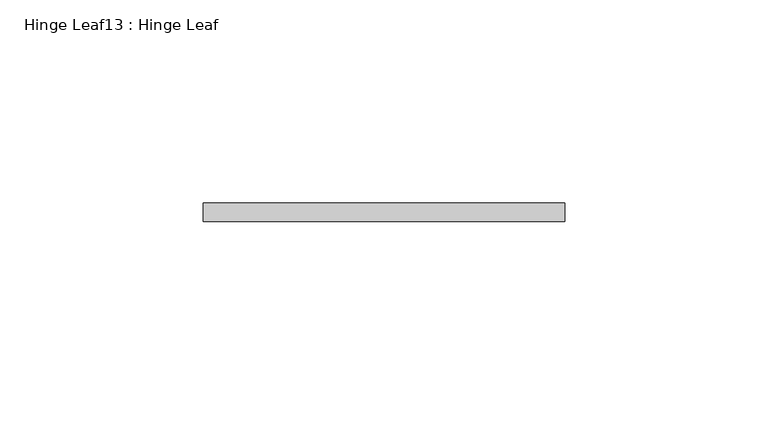
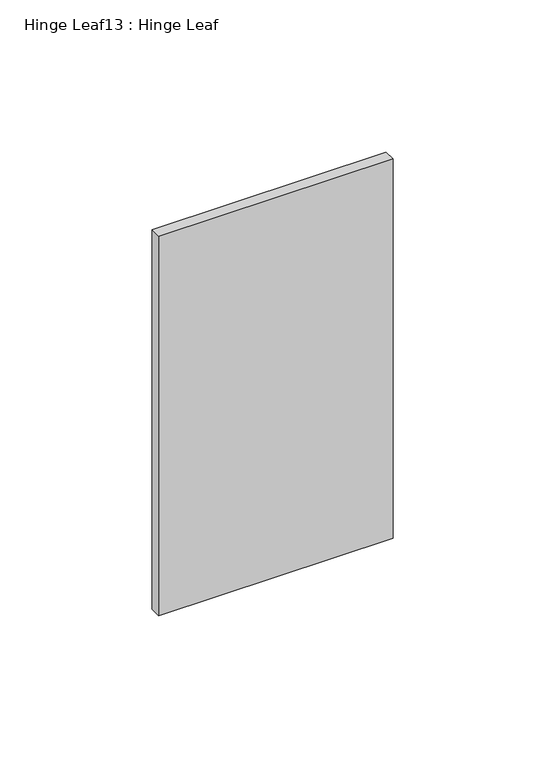
"""IFC4 building model written with IfcOpenShell, lengths in millimetres: proxy geometry, Hinge Leaf13 : Hinge Leaf."""

from ifc_helpers import new_model, si_unit, frame, origin, place, context, project, spatial, polyline, outline, extrude, source, transform, mapped, element, save


def hinge_leaf13_hinge_leaf_bf372cbc(model_context):
    return source(origin(), model_context, "Body", "SweptSolid", [
        extrude(outline(polyline([(587327.7934739, -533988.7163841), (587327.7934739, -533984.1443841), (587416.6934739, -533984.1443841), (587416.6934739, -533988.7163841), (587327.7934739, -533988.7163841)])), frame((0.0, 0.0, 1123.95), z_axis=(0.0, 0.0, 1.0), x_axis=(1.0, 0.0, 0.0)), (0.0, 0.0, 1.0), 152.4),
    ])


if __name__ == "__main__":
    model = new_model("IFC4")
    model_context = context("Model", 3, world=origin())
    ifc_project = project(units=[si_unit("LENGTHUNIT", "METRE", prefix="MILLI")], contexts=[model_context])
    site = spatial("IfcSite", under=ifc_project)
    building = spatial("IfcBuilding", under=site)
    placement = place(None, origin())
    hinge_leaf13_hinge_leaf_shape = hinge_leaf13_hinge_leaf_bf372cbc(model_context)
    element("IfcBuildingElementProxy", 1, Name="Hinge Leaf13 : Hinge Leaf", ObjectType="Hinge Leaf13 : Hinge Leaf", at=placement, inside=building, context=model_context, shape_type="MappedRepresentation", body=[
        mapped(hinge_leaf13_hinge_leaf_shape, transform((0.0, 0.0, 0.0), x_axis=(1.0, 0.0, 0.0), y_axis=(0.0, 1.0, 0.0), z_axis=(0.0, 0.0, 1.0))),
    ])
    save(model, "model.ifc")

# Revit data of these elements
# Element 1 (IfcBuildingElementProxy, "Hinge Leaf13 : Hinge Leaf")
#   Materials on its faces: "6\"X6\" WELD-ON STL BUTT HINGE"
# Materials
#   "6\"X6\" WELD-ON STL BUTT HINGE": class "Metal", colour RGB 189 187 185, transparency 0, Description = "Carbon steel", Cost = 0
